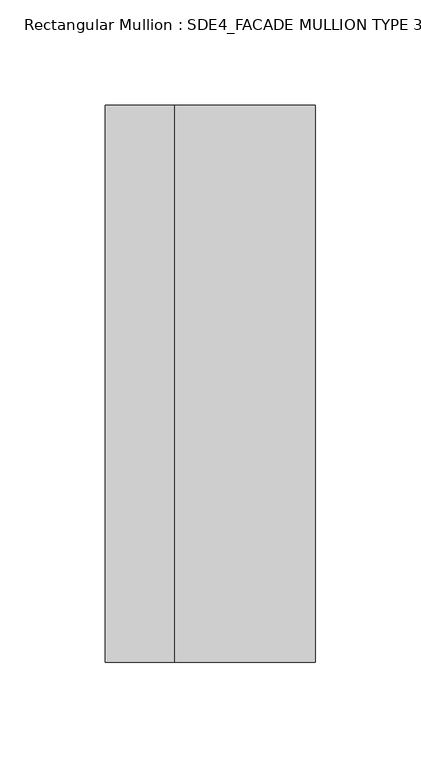
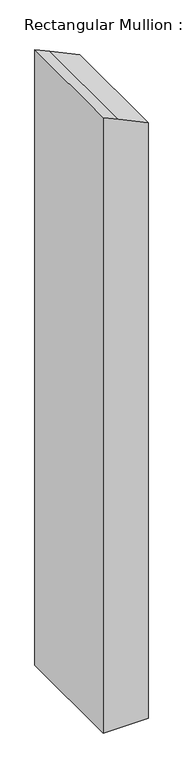
"""IFC4 building model written with IfcOpenShell, lengths in millimetres: member geometry, Rectangular Mullion : SDE4_FACADE MULLION TYPE 3."""

import ifcopenshell
import ifcopenshell.guid

model = None  # the IFC model being written
_history = None  # IfcOwnerHistory: only IFC2X3 demands one
_inside = {}  # id of a spatial element -> (the spatial element, [elements in it])
_under = {}  # id of a project, library or spatial element -> (it, [spatial elements below it])
_declared = {}  # id of a project -> (the project, [libraries it declares])
_typed = {}  # id of a type object -> (the type object, [elements of that type])
_made_of = {}  # id of a material, layer set ... -> (it, [elements and type objects made of it])


def new_model(schema):
    """Start an empty IFC model of exactly this schema.

    Asked for "IFC4X3", IfcOpenShell would pick the latest addendum, in which some entities
    have other attributes; the version numbers below select the first issue.
    IFC2X3 requires an IfcOwnerHistory on every rooted entity: one is made here for all.
    """
    global model, _history
    if schema == "IFC4X3":
        model = ifcopenshell.file(schema_version=(4, 3, 0, 0))
    else:
        model = ifcopenshell.file(schema=schema)
    _inside.clear()
    _under.clear()
    _declared.clear()
    _typed.clear()
    _made_of.clear()
    _history = None
    if model.schema == "IFC2X3":
        org = make("IfcOrganization", Name="unknown")
        user = make(
            "IfcPersonAndOrganization",
            ThePerson=make("IfcPerson", FamilyName="unknown"),
            TheOrganization=org,
        )
        app = make(
            "IfcApplication",
            ApplicationDeveloper=org,
            Version="unknown",
            ApplicationFullName="unknown",
            ApplicationIdentifier="unknown",
        )
        _history = make(
            "IfcOwnerHistory",
            OwningUser=user,
            OwningApplication=app,
            ChangeAction="ADDED",
            CreationDate=0,
        )
    return model


def make(cls, **values):
    """One entity of the class cls with the attributes given. An attribute that is None is left unset."""
    return model.create_entity(
        cls, **{name: value for name, value in values.items() if value is not None}
    )


def rooted(cls, **values):
    """An entity with a GlobalId (a new one), such as an element, a storey or a relation."""
    return make(cls, GlobalId=ifcopenshell.guid.new(), OwnerHistory=_history, **values)


def si_unit(unit_type, name, prefix=None):
    """IfcSIUnit, for example si_unit("LENGTHUNIT", "METRE", prefix="MILLI")."""
    return make("IfcSIUnit", UnitType=unit_type, Prefix=prefix, Name=name)


def assignment(units):
    """IfcUnitAssignment: the units of a project."""
    return None if units is None else make("IfcUnitAssignment", Units=units)


def point(xyz):
    """IfcCartesianPoint."""
    return None if xyz is None else make("IfcCartesianPoint", Coordinates=xyz)


def direction(xyz):
    """IfcDirection."""
    return None if xyz is None else make("IfcDirection", DirectionRatios=xyz)


def frame(location, z_axis=None, x_axis=None):
    """IfcAxis2Placement3D, a coordinate frame: its origin and axes. An axis left out is left unset."""
    return make(
        "IfcAxis2Placement3D",
        Location=point(location),
        Axis=direction(z_axis),
        RefDirection=direction(x_axis),
    )


def origin():
    """The frame at (0, 0, 0) with its axes left unset."""
    return frame((0.0, 0.0, 0.0))


def place(relative_to, where):
    """IfcLocalPlacement: puts the frame where relative to a parent placement (None: the world)."""
    return make(
        "IfcLocalPlacement", PlacementRelTo=relative_to, RelativePlacement=where
    )


def context(
    kind, dimensions, precision=None, world=None, true_north=None, identifier=None
):
    """IfcGeometricRepresentationContext, for example the 3D "Model" context."""
    return make(
        "IfcGeometricRepresentationContext",
        ContextIdentifier=identifier,
        ContextType=kind,
        CoordinateSpaceDimension=dimensions,
        Precision=precision,
        WorldCoordinateSystem=world,
        TrueNorth=true_north,
    )


def project(units=None, contexts=None):
    """IfcProject with its units and contexts."""
    return rooted(
        "IfcProject",
        Name="project",
        RepresentationContexts=contexts,
        UnitsInContext=assignment(units),
    )


def spatial(cls, under=None, at=None, **own):
    """A site, building, storey or space (cls), placed at a placement, below another one or the project."""
    s = rooted(cls, ObjectPlacement=at, **own)
    if under is not None:
        _under.setdefault(under.id(), (under, []))[1].append(s)
    return s


def polyline(points):
    """IfcPolyline through the points."""
    return make("IfcPolyline", Points=[point(p) for p in points])


def outline(outer, holes=None, kind="AREA"):
    """IfcArbitraryClosedProfileDef: a profile drawn as a closed curve; with holes, ...WithVoids."""
    if holes is None:
        return make("IfcArbitraryClosedProfileDef", ProfileType=kind, OuterCurve=outer)
    return make(
        "IfcArbitraryProfileDefWithVoids",
        ProfileType=kind,
        OuterCurve=outer,
        InnerCurves=holes,
    )


def extrude(swept, where, along, depth):
    """IfcExtrudedAreaSolid: the profile swept, set in the frame where, extruded along a direction by depth."""
    return make(
        "IfcExtrudedAreaSolid",
        SweptArea=swept,
        Position=where,
        ExtrudedDirection=direction(along),
        Depth=depth,
    )


def shape(context_of_items, identifier, shape_type, items):
    """IfcShapeRepresentation: the items that make up one representation, for example the "Body"."""
    return make(
        "IfcShapeRepresentation",
        ContextOfItems=context_of_items,
        RepresentationIdentifier=identifier,
        RepresentationType=shape_type,
        Items=items,
    )


def source(mapping_origin, context_of_items, identifier, shape_type, items):
    """IfcRepresentationMap: a shape defined once, which mapped items show again and again."""
    return make(
        "IfcRepresentationMap",
        MappingOrigin=mapping_origin,
        MappedRepresentation=shape(context_of_items, identifier, shape_type, items),
    )


def transform(
    local_origin,
    x_axis=None,
    y_axis=None,
    z_axis=None,
    scale=None,
    scale2=None,
    scale3=None,
    uniform=True,
):
    """IfcCartesianTransformationOperator3D, or its non-uniform kind. x_axis, y_axis, z_axis: its Axis1, 2, 3."""
    if uniform:
        return make(
            "IfcCartesianTransformationOperator3D",
            Axis1=direction(x_axis),
            Axis2=direction(y_axis),
            LocalOrigin=point(local_origin),
            Scale=scale,
            Axis3=direction(z_axis),
        )
    return make(
        "IfcCartesianTransformationOperator3DnonUniform",
        Axis1=direction(x_axis),
        Axis2=direction(y_axis),
        LocalOrigin=point(local_origin),
        Scale=scale,
        Axis3=direction(z_axis),
        Scale2=scale2,
        Scale3=scale3,
    )


def mapped(mapping_source, mapping_target):
    """IfcMappedItem: shows the shape of a source again, moved by a transform."""
    return make(
        "IfcMappedItem", MappingSource=mapping_source, MappingTarget=mapping_target
    )


def made_of(thing, what):
    """Note that an element or type object is made of a material, layer set ...; save() writes the relation."""
    if what is not None:
        _made_of.setdefault(what.id(), (what, []))[1].append(thing)
    return thing


def element(
    cls,
    number,
    at=None,
    inside=None,
    cuts=None,
    type_object=None,
    material=None,
    context=None,
    identifier="Body",
    shape_type=None,
    held_by="IfcProductDefinitionShape",
    body=None,
    shapes=None,
    **own,
):
    """One element of the class cls, such as IfcWall. Its Tag is "e" and its number.

    at: its placement. inside: the storey or other place that contains it. cuts: it is an
    opening in that element (IfcRelVoidsElement). A single representation is given by context,
    identifier, shape_type and body (its items); several are given by shapes. held_by: the class
    of the entity that holds the representations. save() writes the other relations.
    """
    e = rooted(cls, Tag="e%d" % number, ObjectPlacement=at, **own)
    if body is not None:
        shapes = [shape(context, identifier, shape_type, body)]
    if shapes is not None:
        e.Representation = make(held_by, Representations=shapes)
    if inside is not None:
        _inside.setdefault(inside.id(), (inside, []))[1].append(e)
    if cuts is not None:
        rooted(
            "IfcRelVoidsElement", RelatingBuildingElement=cuts, RelatedOpeningElement=e
        )
    if type_object is not None:
        _typed.setdefault(type_object.id(), (type_object, []))[1].append(e)
    return made_of(e, material)


def aggregate(whole, parts):
    """IfcRelAggregates: a whole, such as a stair, and the parts it consists of."""
    return rooted("IfcRelAggregates", RelatingObject=whole, RelatedObjects=parts)


def save(model, path):
    """Write the relations noted so far, then the file.

    IfcRelAggregates (storeys below a building ...), IfcRelContainedInSpatialStructure (elements
    in a storey), IfcRelDefinesByType, IfcRelAssociatesMaterial and IfcRelDeclares: one each for
    every whole, place, type object, material and project.
    """
    for whole, parts in _under.values():
        aggregate(whole, parts)
    for where, things in _inside.values():
        rooted(
            "IfcRelContainedInSpatialStructure",
            RelatedElements=things,
            RelatingStructure=where,
        )
    for kind, things in _typed.values():
        rooted("IfcRelDefinesByType", RelatedObjects=things, RelatingType=kind)
    for what, things in _made_of.values():
        rooted("IfcRelAssociatesMaterial", RelatedObjects=things, RelatingMaterial=what)
    for by, libraries in _declared.values():
        rooted("IfcRelDeclares", RelatingContext=by, RelatedDefinitions=libraries)
    model.write(path)


def rectangular_mullion_sde4_facade_mullion_type_3_b6918dce(model_context):
    return source(origin(), model_context, "Body", "SweptSolid", [
        extrude(outline(polyline([(-67.4504667, 50.0), (-36.2523183, -16.9047158), (-20.8197502, -50.0), (-1475.4067107, -50.0), (-1475.4067107, 50.0), (-67.4504667, 50.0)])), frame((0.0, -132.5, 0.0), z_axis=(0.0, 1.0, 0.0), x_axis=(0.0, 0.0, 1.0)), (0.0, 0.0, 1.0), 265.0),
    ])


if __name__ == "__main__":
    model = new_model("IFC4")
    model_context = context("Model", 3, world=origin())
    ifc_project = project(units=[si_unit("LENGTHUNIT", "METRE", prefix="MILLI")], contexts=[model_context])
    site = spatial("IfcSite", under=ifc_project)
    building = spatial("IfcBuilding", under=site)
    placement = place(None, origin())
    rectangular_mullion_sde4_facade_mullion_type_3_shape = rectangular_mullion_sde4_facade_mullion_type_3_b6918dce(model_context)
    element("IfcMember", 1, ObjectType="Rectangular Mullion : SDE4_FACADE MULLION TYPE 3", at=placement, inside=building, context=model_context, shape_type="MappedRepresentation", body=[
        mapped(rectangular_mullion_sde4_facade_mullion_type_3_shape, transform((0.0, 0.0, 0.0), x_axis=(1.0, 0.0, 0.0), y_axis=(0.0, 1.0, 0.0), z_axis=(0.0, 0.0, 1.0))),
    ])
    save(model, "model.ifc")

# Revit data of these elements
# Type "Rectangular Mullion : SDE4_FACADE MULLION TYPE 3"
#   built-in parameter 1007322 = 0.869423 (stored number, unit not read)
#   built-in parameter 1007321 = 0.164042 (stored number, unit not read)
#   built-in parameter 1007320 = 0.164042 (stored number, unit not read)
